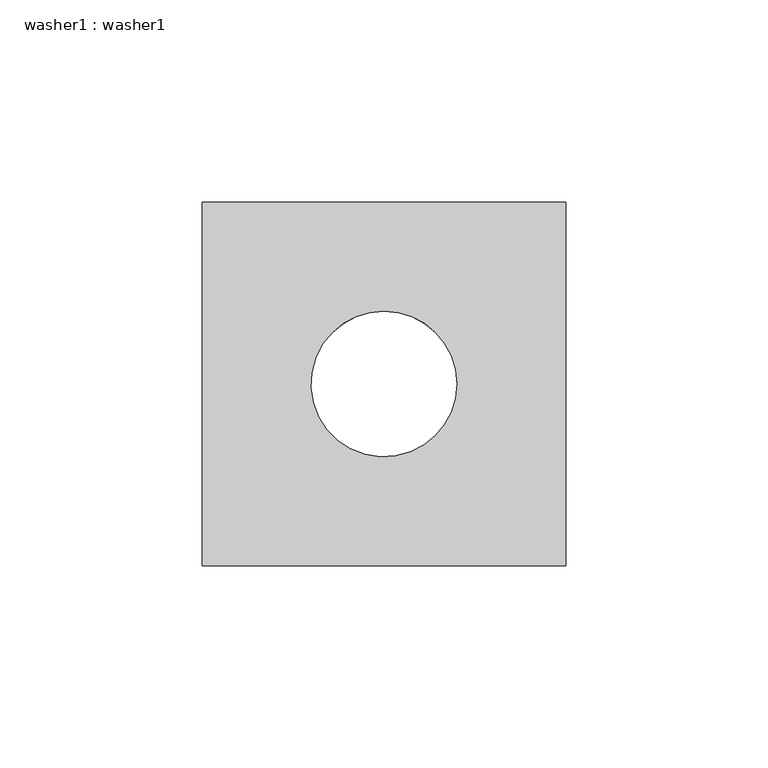
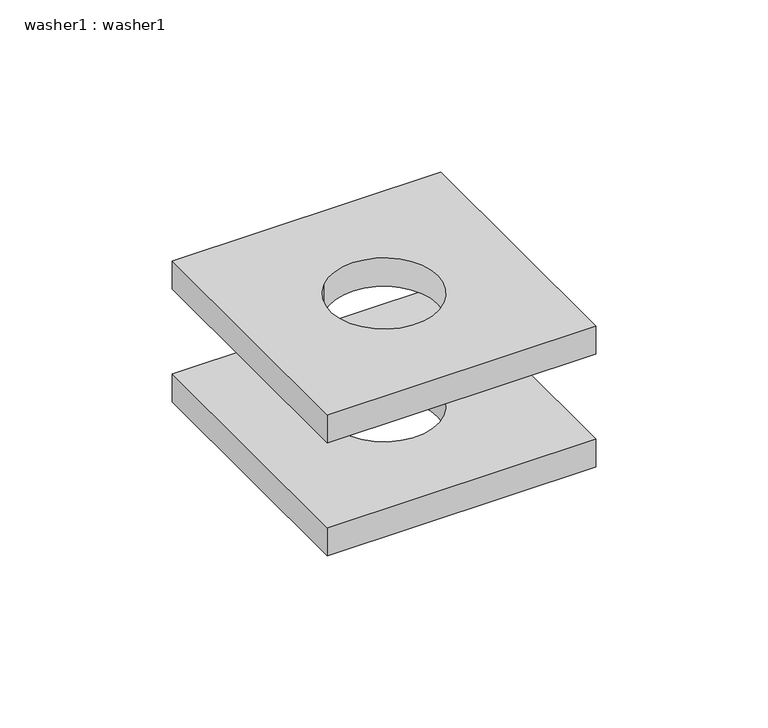
"""IFC4 building model written with IfcOpenShell, lengths in millimetres: fastener geometry, washer1 : washer1."""

from ifc_helpers import new_model, si_unit, point, frame, frame_2d, origin, place, context, project, spatial, polyline, circle_curve, trimmed, segment, composite_curve, outline, extrude, source, transform, mapped, element, save


def washer1_washer1_a000172e(model_context):
    return source(origin(), model_context, "Body", "SweptSolid", [
        extrude(outline(polyline([(-30613.4993654, -7539.0115963), (-30523.4993654, -7539.0115963), (-30523.4993654, -7629.0115963), (-30613.4993654, -7629.0115963), (-30613.4993654, -7539.0115963)]), holes=[composite_curve([segment(trimmed(circle_curve(frame_2d((-30568.4993654, -7584.0115963)), 18.0), [point((-30581.2272874, -7571.2836743))], [point((-30555.7714433, -7596.7395184))], True, "CARTESIAN"), True, "CONTINUOUS"), segment(trimmed(circle_curve(frame_2d((-30568.4993654, -7584.0115963)), 18.0), [point((-30555.7714433, -7596.7395184))], [point((-30581.2272874, -7571.2836743))], True, "CARTESIAN"), True, "CONTINUOUS")], self_intersect=False)]), frame((0.0, 0.0, 150.0), z_axis=(0.0, 0.0, 1.0), x_axis=(1.0, 0.0, 0.0)), (0.0, 0.0, 1.0), 10.0),
        extrude(outline(polyline([(-30613.4993654, -7539.0115963), (-30523.4993654, -7539.0115963), (-30523.4993654, -7629.0115963), (-30613.4993654, -7629.0115963), (-30613.4993654, -7539.0115963)]), holes=[composite_curve([segment(trimmed(circle_curve(frame_2d((-30568.4993654, -7584.0115963)), 18.0), [point((-30581.2272874, -7571.2836743))], [point((-30555.7714433, -7596.7395184))], True, "CARTESIAN"), True, "CONTINUOUS"), segment(trimmed(circle_curve(frame_2d((-30568.4993654, -7584.0115963)), 18.0), [point((-30555.7714433, -7596.7395184))], [point((-30581.2272874, -7571.2836743))], True, "CARTESIAN"), True, "CONTINUOUS")], self_intersect=False)]), frame((0.0, 0.0, 110.0), z_axis=(0.0, 0.0, 1.0), x_axis=(1.0, 0.0, 0.0)), (0.0, 0.0, 1.0), 10.0),
    ])


if __name__ == "__main__":
    model = new_model("IFC4")
    model_context = context("Model", 3, world=origin())
    ifc_project = project(units=[si_unit("LENGTHUNIT", "METRE", prefix="MILLI")], contexts=[model_context])
    site = spatial("IfcSite", under=ifc_project)
    building = spatial("IfcBuilding", under=site)
    placement = place(None, origin())
    washer1_washer1_shape = washer1_washer1_a000172e(model_context)
    element("IfcFastener", 1, ObjectType="washer1 : washer1", at=placement, inside=building, context=model_context, shape_type="MappedRepresentation", body=[
        mapped(washer1_washer1_shape, transform((0.0, 0.0, 0.0), x_axis=(1.0, 0.0, 0.0), y_axis=(0.0, 1.0, 0.0), z_axis=(0.0, 0.0, 1.0))),
    ])
    save(model, "model.ifc")

# Revit data of these elements
# Element 1 (IfcFastener, "washer1 : washer1")
#   Materials on its faces: "A05ZZ166-00007_Roof_Sandiwch Panel_Mineral Wool_non FP"
# Materials
#   "A05ZZ166-00007_Roof_Sandiwch Panel_Mineral Wool_non FP": class "*O 수장공사 - 패널", colour RGB 242 242 242, transparency 0, Keynote = "OJ4", Description = "샌드위치패널", W00) Work Master Code = "A05ZZ166-00007", W01) Work Master_Lv1 = "Cladding Work", W02) Work Master_Lv2 = "Sandwich Panel", W03) Work Master_Spec.1 = "Corrugated Galvanized Steel Sheet Sandwich Panel, Fire Protective Rating: N/A", W04) Work Master_Spec.2 = "Mineral Wool", W05) Work Master_Spec.3 = "w/ Accessories, Flashing", W06) Work Master_Spec.4 = "100mm≤THK<150mm", Cost = 0
